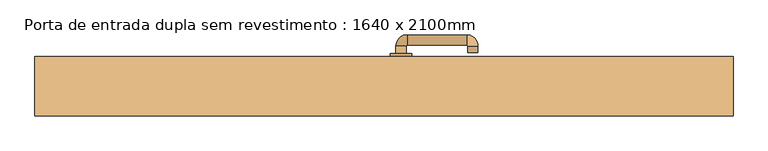
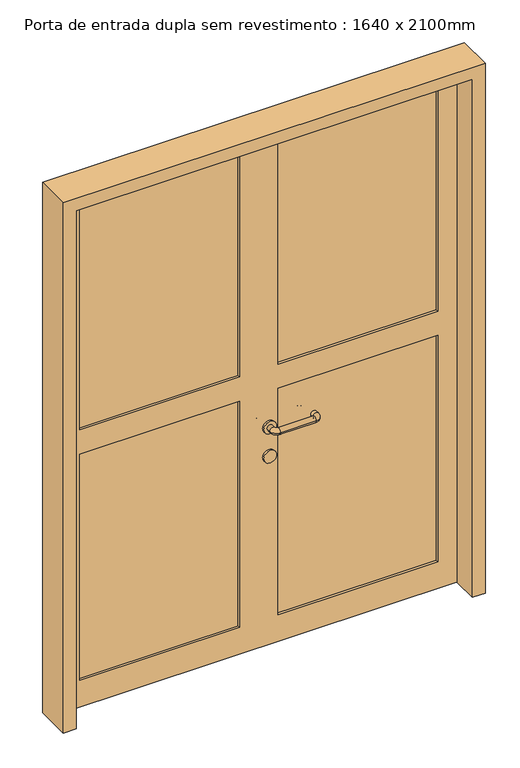
"""IFC4 building model written with IfcOpenShell, lengths in millimetres: door geometry, Porta de entrada dupla sem revestimento : 1640 x 2100mm."""

from ifc_helpers import new_model, si_unit, point, frame, frame_2d, origin, place, context, project, spatial, polyline, circle_curve, ellipse_curve, trimmed, segment, composite_curve, outline, extrude, faceted_brep, source, transform, mapped, element, save
from ifc_brep_helpers import plane_surface, cylinder_surface, revolved_surface, advanced_brep


def porta_de_entrada_dupla_sem_revestimento_1640_x_2100mm_154eaa20(model_context):
    return source(origin(), model_context, "Body", "SolidModel", [
        advanced_brep(
        [(52.0, 27.0, 900.0), (28.0, 27.0, 900.0), (28.0, 10.0, 900.0), (52.0, 10.0, 900.0), (55.0, -17.0, 900.0), (55.0, 7.0, 900.0), (195.0, -17.0, 900.0), (195.0, 7.0, 900.0), (222.0, 10.0, 900.0), (198.0, 10.0, 900.0), (198.0, 25.0, 900.0), (222.0, 25.0, 900.0)],
        [
            (0, 1, circle_curve(frame((40.0, 27.0, 900.0), z_axis=(0.0, 1.0, 0.0), x_axis=(-1.0, 0.0, 0.0)), 12.0)),
            (1, 0, circle_curve(frame((40.0, 27.0, 900.0), z_axis=(0.0, 1.0, 0.0), x_axis=(-1.0, 0.0, 0.0)), 12.0)),
            (1, 2),
            (2, 3, circle_curve(frame((40.0, 10.0, 900.0), z_axis=(0.0, 1.0, 0.0), x_axis=(-1.0, 0.0, 0.0)), 12.0)),
            (3, 0),
            (3, 2, circle_curve(frame((40.0, 10.0, 900.0), z_axis=(0.0, 1.0, 0.0), x_axis=(-1.0, 0.0, 0.0)), 12.0)),
            (4, 5, circle_curve(frame((55.0, -5.0, 900.0), z_axis=(-1.0, 0.0, 0.0), x_axis=(0.0, -1.0, 0.0)), 12.0)),
            (5, 3, circle_curve(frame((55.0, 10.0, 900.0), z_axis=(0.0, 0.0, -1.0), x_axis=(-1.0, 0.0, 0.0)), 3.0)),
            (2, 4, circle_curve(frame((55.0, 10.0, 900.0), z_axis=(0.0, 0.0, 1.0), x_axis=(-1.0, 0.0, 0.0)), 27.0)),
            (5, 4, circle_curve(frame((55.0, -5.0, 900.0), z_axis=(-1.0, 0.0, 0.0), x_axis=(0.0, -1.0, 0.0)), 12.0)),
            (4, 6),
            (6, 7, circle_curve(frame((195.0, -5.0, 900.0), z_axis=(-1.0, 0.0, 0.0), x_axis=(0.0, -1.0, 0.0)), 12.0)),
            (7, 5),
            (7, 6, circle_curve(frame((195.0, -5.0, 900.0), z_axis=(-1.0, 0.0, 0.0), x_axis=(0.0, -1.0, 0.0)), 12.0)),
            (8, 9, circle_curve(frame((210.0, 10.0, 900.0), z_axis=(0.0, -1.0, 0.0), x_axis=(1.0, 0.0, 0.0)), 12.0)),
            (9, 7, circle_curve(frame((195.0, 10.0, 900.0), z_axis=(0.0, 0.0, -1.0), x_axis=(0.0, -1.0, 0.0)), 3.0)),
            (6, 8, circle_curve(frame((195.0, 10.0, 900.0), z_axis=(0.0, 0.0, 1.0), x_axis=(0.0, -1.0, 0.0)), 27.0)),
            (9, 8, circle_curve(frame((210.0, 10.0, 900.0), z_axis=(0.0, -1.0, 0.0), x_axis=(1.0, 0.0, 0.0)), 12.0)),
            (10, 11, circle_curve(frame((210.0, 25.0, 900.0), z_axis=(0.0, 1.0, 0.0), x_axis=(1.0, 0.0, 0.0)), 12.0)),
            (11, 10, circle_curve(frame((210.0, 25.0, 900.0), z_axis=(0.0, 1.0, 0.0), x_axis=(1.0, 0.0, 0.0)), 12.0)),
            (8, 11),
            (10, 9),
        ],
        [
            plane_surface(frame((-802.0, 27.0, 1730.0), z_axis=(0.0, 1.0, 0.0), x_axis=(0.0, 0.0, 1.0))),
            cylinder_surface(frame((40.0, 27.0, 900.0), z_axis=(0.0, 1.0, 0.0), x_axis=(-1.0, 0.0, 0.0)), 12.0),
            revolved_surface(trimmed(ellipse_curve(frame((40.0, 10.0, 900.0), z_axis=(0.0, -1.0, 0.0), x_axis=(-1.0, 0.0, 0.0)), 12.0, 12.0), [point((52.0, 10.0, 900.0))], [point((28.0, 10.0, 900.0))], True, "CARTESIAN"), (55.0, 10.0, 1730.0), (0.0, 0.0, -1.0)),
            revolved_surface(trimmed(ellipse_curve(frame((40.0, 10.0, 900.0), z_axis=(0.0, -1.0, 0.0), x_axis=(-1.0, 0.0, 0.0)), 12.0, 12.0), [point((28.0, 10.0, 900.0))], [point((52.0, 10.0, 900.0))], True, "CARTESIAN"), (55.0, 10.0, 1730.0), (0.0, 0.0, -1.0)),
            cylinder_surface(frame((55.0, -5.0, 900.0), z_axis=(-1.0, 0.0, 0.0), x_axis=(0.0, -1.0, 0.0)), 12.0),
            revolved_surface(trimmed(ellipse_curve(frame((195.0, -5.0, 900.0), z_axis=(1.0, 0.0, 0.0), x_axis=(0.0, -1.0, 0.0)), 12.0, 12.0), [point((195.0, 7.0, 900.0))], [point((195.0, -17.0, 900.0))], True, "CARTESIAN"), (195.0, 10.0, 1730.0), (0.0, 0.0, -1.0)),
            revolved_surface(trimmed(ellipse_curve(frame((195.0, -5.0, 900.0), z_axis=(1.0, 0.0, 0.0), x_axis=(0.0, -1.0, 0.0)), 12.0, 12.0), [point((195.0, -17.0, 900.0))], [point((195.0, 7.0, 900.0))], True, "CARTESIAN"), (195.0, 10.0, 1730.0), (0.0, 0.0, -1.0)),
            plane_surface(frame((-632.0, 25.0, 1730.0), z_axis=(0.0, 1.0, 0.0), x_axis=(0.0, 0.0, -1.0))),
            cylinder_surface(frame((210.0, 10.0, 900.0), z_axis=(0.0, -1.0, 0.0), x_axis=(1.0, 0.0, 0.0)), 12.0),
        ],
        [
            (0, [[1, 2]]),
            (1, [[3, 4, 5, -2]]),
            (1, [[-5, 6, -3, -1]]),
            (2, [[7, 8, -4, 9]]),
            (3, [[10, -9, -6, -8]]),
            (4, [[11, 12, 13, -7]]),
            (4, [[-13, 14, -11, -10]]),
            (5, [[15, 16, -12, 17]]),
            (6, [[18, -17, -14, -16]]),
            (7, [[19, 20]]),
            (8, [[21, -19, 22, -15]]),
            (8, [[-22, -20, -21, -18]]),
        ],
    ),
        extrude(outline(composite_curve([segment(trimmed(circle_curve(frame_2d((780.0, 40.0)), 25.0), [point((780.0, 15.0))], [point((780.0, 65.0))], False, "CARTESIAN"), True, "CONTINUOUS"), segment(trimmed(circle_curve(frame_2d((780.0, 40.0)), 25.0), [point((780.0, 65.0))], [point((780.0, 15.0))], False, "CARTESIAN"), True, "CONTINUOUS")], self_intersect=False)), frame((0.0, 27.0, 0.0), z_axis=(0.0, 1.0, 0.0), x_axis=(0.0, 0.0, 1.0)), (0.0, 0.0, 1.0), 8.0),
        extrude(outline(composite_curve([segment(trimmed(circle_curve(frame_2d((900.0, 40.0)), 25.0), [point((900.0, 15.0))], [point((900.0, 65.0))], False, "CARTESIAN"), True, "CONTINUOUS"), segment(trimmed(circle_curve(frame_2d((900.0, 40.0)), 25.0), [point((900.0, 65.0))], [point((900.0, 15.0))], False, "CARTESIAN"), True, "CONTINUOUS")], self_intersect=False)), frame((0.0, 27.0, 0.0), z_axis=(0.0, 1.0, 0.0), x_axis=(0.0, 0.0, 1.0)), (0.0, 0.0, 1.0), 8.0),
        advanced_brep(
        [(28.0, 78.0, 900.0), (52.0, 78.0, 900.0), (52.0, 95.0, 900.0), (28.0, 95.0, 900.0), (55.0, 98.0, 900.0), (55.0, 122.0, 900.0), (195.0, 98.0, 900.0), (195.0, 122.0, 900.0), (198.0, 95.0, 900.0), (222.0, 95.0, 900.0), (222.0, 80.0, 900.0), (198.0, 80.0, 900.0)],
        [
            (0, 1, circle_curve(frame((40.0, 78.0, 900.0), z_axis=(0.0, -1.0, 0.0), x_axis=(1.0, 0.0, 0.0)), 12.0)),
            (1, 0, circle_curve(frame((40.0, 78.0, 900.0), z_axis=(0.0, -1.0, 0.0), x_axis=(1.0, 0.0, 0.0)), 12.0)),
            (1, 2),
            (2, 3, circle_curve(frame((40.0, 95.0, 900.0), z_axis=(0.0, -1.0, 0.0), x_axis=(1.0, 0.0, 0.0)), 12.0)),
            (3, 0),
            (3, 2, circle_curve(frame((40.0, 95.0, 900.0), z_axis=(0.0, -1.0, 0.0), x_axis=(1.0, 0.0, 0.0)), 12.0)),
            (4, 5, circle_curve(frame((55.0, 110.0, 900.0), z_axis=(-1.0, 0.0, 0.0), x_axis=(0.0, -1.0, 0.0)), 12.0)),
            (5, 3, circle_curve(frame((55.0, 95.0, 900.0), z_axis=(0.0, 0.0, 1.0), x_axis=(-1.0, 0.0, 0.0)), 27.0)),
            (2, 4, circle_curve(frame((55.0, 95.0, 900.0), z_axis=(0.0, 0.0, -1.0), x_axis=(-1.0, 0.0, 0.0)), 3.0)),
            (5, 4, circle_curve(frame((55.0, 110.0, 900.0), z_axis=(-1.0, 0.0, 0.0), x_axis=(0.0, -1.0, 0.0)), 12.0)),
            (4, 6),
            (6, 7, circle_curve(frame((195.0, 110.0, 900.0), z_axis=(-1.0, 0.0, 0.0), x_axis=(0.0, -1.0, 0.0)), 12.0)),
            (7, 5),
            (7, 6, circle_curve(frame((195.0, 110.0, 900.0), z_axis=(-1.0, 0.0, 0.0), x_axis=(0.0, -1.0, 0.0)), 12.0)),
            (8, 9, circle_curve(frame((210.0, 95.0, 900.0), z_axis=(0.0, 1.0, 0.0), x_axis=(-1.0, 0.0, 0.0)), 12.0)),
            (9, 7, circle_curve(frame((195.0, 95.0, 900.0), z_axis=(0.0, 0.0, 1.0), x_axis=(0.0, 1.0, 0.0)), 27.0)),
            (6, 8, circle_curve(frame((195.0, 95.0, 900.0), z_axis=(0.0, 0.0, -1.0), x_axis=(0.0, 1.0, 0.0)), 3.0)),
            (9, 8, circle_curve(frame((210.0, 95.0, 900.0), z_axis=(0.0, 1.0, 0.0), x_axis=(-1.0, 0.0, 0.0)), 12.0)),
            (10, 11, circle_curve(frame((210.0, 80.0, 900.0), z_axis=(0.0, -1.0, 0.0), x_axis=(-1.0, 0.0, 0.0)), 12.0)),
            (11, 10, circle_curve(frame((210.0, 80.0, 900.0), z_axis=(0.0, -1.0, 0.0), x_axis=(-1.0, 0.0, 0.0)), 12.0)),
            (8, 11),
            (10, 9),
        ],
        [
            plane_surface(frame((-802.0, 78.0, 1730.0), z_axis=(0.0, -1.0, 0.0), x_axis=(0.0, 0.0, -1.0))),
            cylinder_surface(frame((40.0, 78.0, 900.0), z_axis=(0.0, -1.0, 0.0), x_axis=(1.0, 0.0, 0.0)), 12.0),
            revolved_surface(trimmed(ellipse_curve(frame((40.0, 95.0, 900.0), z_axis=(0.0, 1.0, 0.0), x_axis=(1.0, 0.0, 0.0)), 12.0, 12.0), [point((28.0, 95.0, 900.0))], [point((52.0, 95.0, 900.0))], True, "CARTESIAN"), (55.0, 95.0, 1730.0), (0.0, 0.0, 1.0)),
            revolved_surface(trimmed(ellipse_curve(frame((40.0, 95.0, 900.0), z_axis=(0.0, 1.0, 0.0), x_axis=(1.0, 0.0, 0.0)), 12.0, 12.0), [point((52.0, 95.0, 900.0))], [point((28.0, 95.0, 900.0))], True, "CARTESIAN"), (55.0, 95.0, 1730.0), (0.0, 0.0, 1.0)),
            cylinder_surface(frame((55.0, 110.0, 900.0), z_axis=(-1.0, 0.0, 0.0), x_axis=(0.0, -1.0, 0.0)), 12.0),
            revolved_surface(trimmed(ellipse_curve(frame((195.0, 110.0, 900.0), z_axis=(1.0, 0.0, 0.0), x_axis=(0.0, -1.0, 0.0)), 12.0, 12.0), [point((195.0, 122.0, 900.0))], [point((195.0, 98.0, 900.0))], True, "CARTESIAN"), (195.0, 95.0, 1730.0), (0.0, 0.0, 1.0)),
            revolved_surface(trimmed(ellipse_curve(frame((195.0, 110.0, 900.0), z_axis=(1.0, 0.0, 0.0), x_axis=(0.0, -1.0, 0.0)), 12.0, 12.0), [point((195.0, 98.0, 900.0))], [point((195.0, 122.0, 900.0))], True, "CARTESIAN"), (195.0, 95.0, 1730.0), (0.0, 0.0, 1.0)),
            plane_surface(frame((-632.0, 80.0, 1730.0), z_axis=(0.0, -1.0, 0.0), x_axis=(0.0, 0.0, 1.0))),
            cylinder_surface(frame((210.0, 95.0, 900.0), z_axis=(0.0, 1.0, 0.0), x_axis=(-1.0, 0.0, 0.0)), 12.0),
        ],
        [
            (0, [[1, 2]]),
            (1, [[3, 4, 5, -2]]),
            (1, [[-5, 6, -3, -1]]),
            (2, [[7, 8, -4, 9]]),
            (3, [[10, -9, -6, -8]]),
            (4, [[11, 12, 13, -7]]),
            (4, [[-13, 14, -11, -10]]),
            (5, [[15, 16, -12, 17]]),
            (6, [[18, -17, -14, -16]]),
            (7, [[19, 20]]),
            (8, [[21, -19, 22, -15]]),
            (8, [[-22, -20, -21, -18]]),
        ],
    ),
        extrude(outline(composite_curve([segment(trimmed(circle_curve(frame_2d((780.0, 40.0)), 25.0), [point((780.0, 15.0))], [point((780.0, 65.0))], False, "CARTESIAN"), True, "CONTINUOUS"), segment(trimmed(circle_curve(frame_2d((780.0, 40.0)), 25.0), [point((780.0, 65.0))], [point((780.0, 15.0))], False, "CARTESIAN"), True, "CONTINUOUS")], self_intersect=False)), frame((0.0, 70.0, 0.0), z_axis=(0.0, 1.0, 0.0), x_axis=(0.0, 0.0, 1.0)), (0.0, 0.0, 1.0), 8.0),
        extrude(outline(composite_curve([segment(trimmed(circle_curve(frame_2d((900.0, 40.0)), 25.0), [point((900.0, 15.0))], [point((900.0, 65.0))], False, "CARTESIAN"), True, "CONTINUOUS"), segment(trimmed(circle_curve(frame_2d((900.0, 40.0)), 25.0), [point((900.0, 65.0))], [point((900.0, 15.0))], False, "CARTESIAN"), True, "CONTINUOUS")], self_intersect=False)), frame((0.0, 70.0, 0.0), z_axis=(0.0, 1.0, 0.0), x_axis=(0.0, 0.0, 1.0)), (0.0, 0.0, 1.0), 8.0),
        extrude(outline(polyline([(-740.0, 45.5), (-740.0, 59.5), (740.0, 59.5), (740.0, 45.5), (-740.0, 45.5)])), frame((0.0, 0.0, 70.0), z_axis=(0.0, 0.0, 1.0), x_axis=(1.0, 0.0, 0.0)), (0.0, 0.0, 1.0), 1015.0),
        extrude(outline(polyline([(-740.0, 45.5), (-740.0, 59.5), (740.0, 59.5), (740.0, 45.5), (-740.0, 45.5)])), frame((0.0, 0.0, 1105.0), z_axis=(0.0, 0.0, 1.0), x_axis=(1.0, 0.0, 0.0)), (0.0, 0.0, 1.0), 1000.0),
        extrude(outline(polyline([(-740.0, 45.5), (-740.0, 59.5), (740.0, 59.5), (740.0, 45.5), (-740.0, 45.5)])), frame((0.0, 0.0, 70.0), z_axis=(0.0, 0.0, 1.0), x_axis=(1.0, 0.0, 0.0)), (0.0, 0.0, 1.0), 1015.0),
        extrude(outline(polyline([(-740.0, 45.5), (-740.0, 59.5), (740.0, 59.5), (740.0, 45.5), (-740.0, 45.5)])), frame((0.0, 0.0, 1105.0), z_axis=(0.0, 0.0, 1.0), x_axis=(1.0, 0.0, 0.0)), (0.0, 0.0, 1.0), 1000.0),
        faceted_brep([(-825.0, -70.0, 0.0), (-825.0, 70.0, 0.0), (-785.0, 70.0, 0.0), (-785.0, 32.0, 0.0), (-775.0, 32.0, 0.0), (-775.0, -70.0, 0.0), (-775.0, -70.0, 2140.0), (775.0, -70.0, 2140.0), (775.0, -70.0, 0.0), (825.0, -70.0, 0.0), (825.0, -70.0, 2190.0), (-825.0, -70.0, 2190.0), (-775.0, 32.0, 2140.0), (-785.0, 32.0, 2150.0), (785.0, 32.0, 2150.0), (785.0, 32.0, 0.0), (775.0, 32.0, 0.0), (775.0, 32.0, 2140.0), (-785.0, 70.0, 2150.0), (-825.0, 70.0, 2190.0), (825.0, 70.0, 2190.0), (825.0, 70.0, 0.0), (785.0, 70.0, 0.0), (785.0, 70.0, 2150.0)], [[[0, 1, 2, 3, 4, 5]], [[5, 6, 7, 8, 9, 10, 11, 0]], [[4, 12, 6, 5]], [[3, 13, 14, 15, 16, 17, 12, 4]], [[2, 18, 13, 3]], [[1, 19, 20, 21, 22, 23, 18, 2]], [[0, 11, 19, 1]], [[10, 9, 21, 20]], [[9, 8, 16, 15, 22, 21]], [[17, 16, 8, 7]], [[23, 22, 15, 14]], [[12, 17, 7, 6]], [[18, 23, 14, 13]], [[11, 10, 20, 19]]]),
        extrude(outline(polyline([(2150.0, -785.0), (0.0, -785.0), (0.0, 785.0), (2150.0, 785.0), (2150.0, -785.0)]), holes=[polyline([(1045.0, 700.0), (110.0, 700.0), (110.0, 75.0), (1045.0, 75.0), (1045.0, 700.0)]), polyline([(2065.0, 75.0), (2065.0, 700.0), (1145.0, 700.0), (1145.0, 75.0), (2065.0, 75.0)]), polyline([(1145.0, -700.0), (2065.0, -700.0), (2065.0, -75.0), (1145.0, -75.0), (1145.0, -700.0)]), polyline([(110.0, -75.0), (110.0, -700.0), (1045.0, -700.0), (1045.0, -75.0), (110.0, -75.0)])]), frame((0.0, 35.0, 0.0), z_axis=(0.0, 1.0, 0.0), x_axis=(0.0, 0.0, 1.0)), (0.0, 0.0, 1.0), 35.0),
    ])


if __name__ == "__main__":
    model = new_model("IFC4")
    model_context = context("Model", 3, world=origin())
    ifc_project = project(units=[si_unit("LENGTHUNIT", "METRE", prefix="MILLI")], contexts=[model_context])
    site = spatial("IfcSite", under=ifc_project)
    building = spatial("IfcBuilding", under=site)
    placement = place(None, origin())
    porta_de_entrada_dupla_sem_revestimento_1640_x_2100mm_shape = porta_de_entrada_dupla_sem_revestimento_1640_x_2100mm_154eaa20(model_context)
    element("IfcDoor", 1, ObjectType="Porta de entrada dupla sem revestimento : 1640 x 2100mm", at=placement, inside=building, context=model_context, shape_type="MappedRepresentation", body=[
        mapped(porta_de_entrada_dupla_sem_revestimento_1640_x_2100mm_shape, transform((0.0, 0.0, 0.0), x_axis=(1.0, 0.0, 0.0), y_axis=(0.0, 1.0, 0.0), z_axis=(0.0, 0.0, 1.0))),
    ])
    save(model, "model.ifc")

# Revit data of these elements
# Type "Porta de entrada dupla sem revestimento : 1640 x 2100mm"
#   Type Mark = "150"
#   Construction Type Id = "MPORTA"
#   Analytic Construction = "Metal"
#   W2 = 0.825 m
#   W1 = 1.570 m
#   Thickness = 0.035 m
#   Rough Width = 1.650 m
#   Rough Height = 2.190 m
#   Largura da moldura do painel = 0.075 m
#   Heat Transfer Coefficient (U) = 3.7021 W/(m²·K)
#   Largura da estrutura = 0.050 m
#   Height = 2.190 m
#   Width = 1.650 m
#   Define Thermal Properties by = 1
#   Function = 1
#   Material do painel = none
#   Material do puxador = none
#   Vidro = none
#   Material da moldura = none
#   Visual Light Transmittance = 0
#   Solar Heat Gain Coefficient = 0
#   Wall Closure = (empty or 0)
# Element 1 (IfcDoor, "Porta de entrada dupla sem revestimento : 1640 x 2100mm")
#   Materials on its faces: "Vidro 10mm"
# Materials
#   "Vidro 10mm": class "Glass", colour RGB 225 255 255, transparency 0.74, Cost = 0
